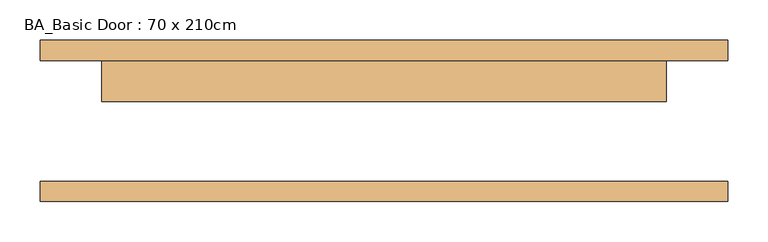
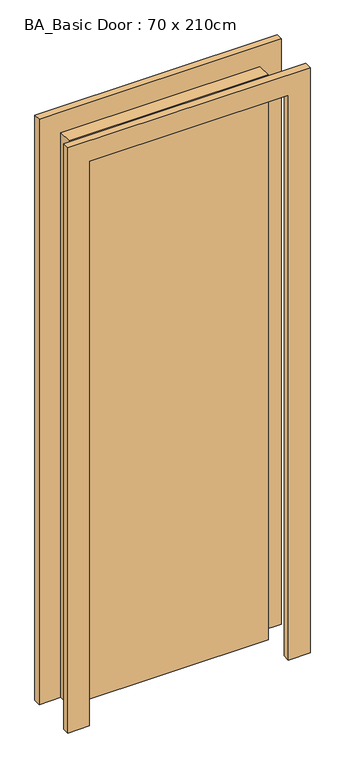
"""IFC4 building model written with IfcOpenShell, lengths in millimetres: door geometry, BA_Basic Door : 70 x 210cm."""

from ifc_helpers import new_model, si_unit, frame, origin, origin_with_axes, place, context, project, spatial, polyline, outline, extrude, source, transform, mapped, element, save


def ba_basic_door_70_x_210cm_b6d038f8(model_context):
    return source(origin(), model_context, "Body", "SweptSolid", [
        extrude(outline(polyline([(350.0, 24.0), (-350.0, 24.0), (-350.0, 75.0), (350.0, 75.0), (350.0, 24.0)])), origin_with_axes(), (0.0, 0.0, 1.0), 2100.0),
        extrude(outline(polyline([(2176.0, -426.0), (0.0, -426.0), (0.0, -350.0), (2100.0, -350.0), (2100.0, 350.0), (0.0, 350.0), (0.0, 426.0), (2176.0, 426.0), (2176.0, -426.0)])), frame((0.0, 75.0, 0.0), z_axis=(0.0, 1.0, 0.0), x_axis=(0.0, 0.0, 1.0)), (0.0, 0.0, 1.0), 25.0),
        extrude(outline(polyline([(2176.0, 426.0), (2176.0, -426.0), (0.0, -426.0), (0.0, -350.0), (2100.0, -350.0), (2100.0, 350.0), (0.0, 350.0), (0.0, 426.0), (2176.0, 426.0)])), frame((0.0, -100.0, 0.0), z_axis=(0.0, 1.0, 0.0), x_axis=(0.0, 0.0, 1.0)), (0.0, 0.0, 1.0), 25.0),
    ])


if __name__ == "__main__":
    model = new_model("IFC4")
    model_context = context("Model", 3, world=origin())
    ifc_project = project(units=[si_unit("LENGTHUNIT", "METRE", prefix="MILLI")], contexts=[model_context])
    site = spatial("IfcSite", under=ifc_project)
    building = spatial("IfcBuilding", under=site)
    placement = place(None, origin())
    ba_basic_door_70_x_210cm_shape = ba_basic_door_70_x_210cm_b6d038f8(model_context)
    element("IfcDoor", 1, ObjectType="BA_Basic Door : 70 x 210cm", at=placement, inside=building, context=model_context, shape_type="MappedRepresentation", body=[
        mapped(ba_basic_door_70_x_210cm_shape, transform((0.0, 0.0, 0.0), x_axis=(1.0, 0.0, 0.0), y_axis=(0.0, 1.0, 0.0), z_axis=(0.0, 0.0, 1.0))),
    ])
    save(model, "model.ifc")

# Revit data of these elements
# Type "BA_Basic Door : 70 x 210cm"
#   Type Mark = "42"
#   Construction Type Id = "MDOOR"
#   Analytic Construction = "Metal"
#   Window height [instance default] = 1000 mm
#   Thickness = 51 mm
#   Thermal Resistance (R) = 0.270117 (m²·K)/W
#   Cut [instance default] = -100 mm
#   Heat Transfer Coefficient (U) = 3.7021 W/(m²·K)
#   Height = 2100 mm
#   Trim Projection Ext = 25 mm
#   Trim Projection Int = 25 mm
#   Trim Width = 76 mm
#   Width = 700 mm
#   Door window [instance default] = no
#   Define Thermal Properties by = 1
#   Door Material = Default
#   Frame Material = Default
#   Visual Light Transmittance = 0
#   Solar Heat Gain Coefficient = 0
#   Function = (empty or 0)
#   Wall Closure = (empty or 0)
# Element 1 (IfcDoor, "BA_Basic Door : 70 x 210cm")
#   Materials on its faces: "Default"
# Materials
#   "Default": class "Generic", colour RGB 255 255 255, transparency 0, Cost = 0
